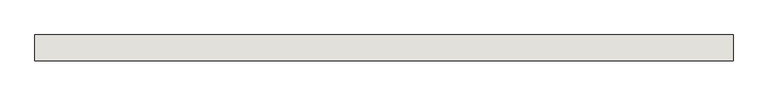
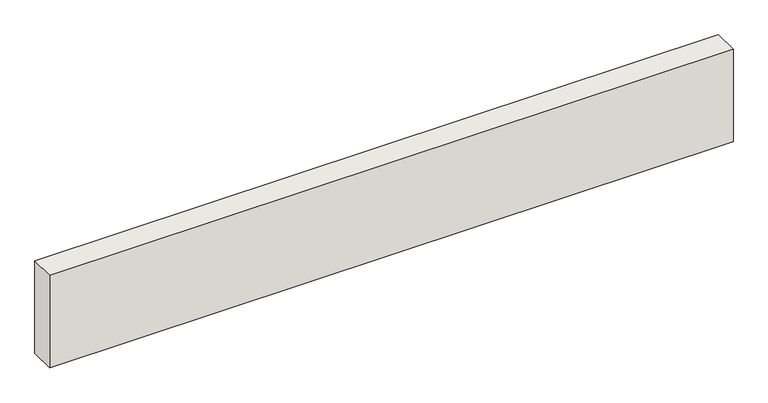
"""IFC4 building model written with IfcOpenShell, lengths in millimetres: wall geometry, 0_3d."""

from ifc_helpers import new_model, si_unit, frame, origin, place, context, project, spatial, polyline, outline, extrude, source, transform, mapped, element, save


def wall_ceec1391(model_context):
    return source(origin(), model_context, "Body", "SweptSolid", [
        extrude(outline(polyline([(2100.0, 0.0), (0.0, 0.0), (0.0, 78.0), (2100.0, 78.0), (2100.0, 0.0)])), frame((0.0, 0.0, 2580.0), z_axis=(0.0, 0.0, 1.0), x_axis=(1.0, 0.0, 0.0)), (0.0, 0.0, 1.0), 300.0),
    ])


if __name__ == "__main__":
    model = new_model("IFC4")
    model_context = context("Model", 3, world=origin())
    ifc_project = project(units=[si_unit("LENGTHUNIT", "METRE", prefix="MILLI")], contexts=[model_context])
    site = spatial("IfcSite", under=ifc_project)
    building = spatial("IfcBuilding", under=site)
    placement = place(None, origin())
    wall_shape = wall_ceec1391(model_context)
    element("IfcWall", 1, ObjectType="0_3d", at=placement, inside=building, context=model_context, shape_type="MappedRepresentation", body=[
        mapped(wall_shape, transform((0.0, 0.0, 0.0), x_axis=(1.0, 0.0, 0.0), y_axis=(0.0, 1.0, 0.0), z_axis=(0.0, 0.0, 1.0))),
    ])
    save(model, "model.ifc")

# Revit data of these elements
# Element 1 (IfcWall, "0_3d")
#   Materials on its faces: "glas"
# Materials
#   "glas": class "Unassigned", colour RGB 250 253 254, transparency 0.95
